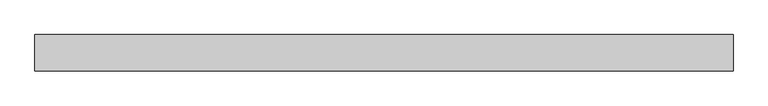
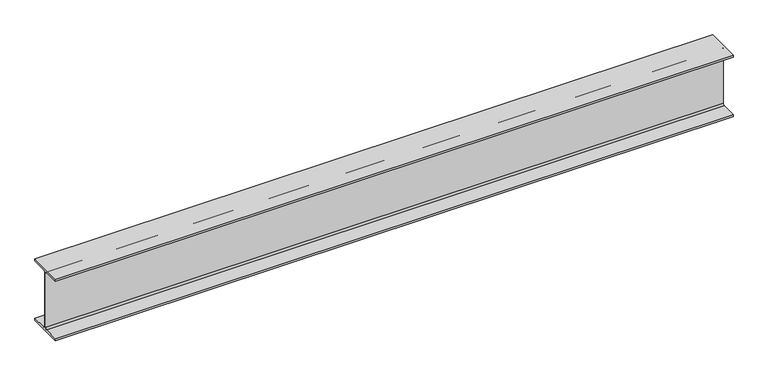
"""IFC4 building model written with IfcOpenShell, lengths in millimetres: beam geometry, Steel Beam_H-KSD3502 : H_SB_ASB_H-200x200x8x12."""

import ifcopenshell
import ifcopenshell.guid

model = None  # the IFC model being written
_history = None  # IfcOwnerHistory: only IFC2X3 demands one
_inside = {}  # id of a spatial element -> (the spatial element, [elements in it])
_under = {}  # id of a project, library or spatial element -> (it, [spatial elements below it])
_declared = {}  # id of a project -> (the project, [libraries it declares])
_typed = {}  # id of a type object -> (the type object, [elements of that type])
_made_of = {}  # id of a material, layer set ... -> (it, [elements and type objects made of it])


def new_model(schema):
    """Start an empty IFC model of exactly this schema.

    Asked for "IFC4X3", IfcOpenShell would pick the latest addendum, in which some entities
    have other attributes; the version numbers below select the first issue.
    IFC2X3 requires an IfcOwnerHistory on every rooted entity: one is made here for all.
    """
    global model, _history
    if schema == "IFC4X3":
        model = ifcopenshell.file(schema_version=(4, 3, 0, 0))
    else:
        model = ifcopenshell.file(schema=schema)
    _inside.clear()
    _under.clear()
    _declared.clear()
    _typed.clear()
    _made_of.clear()
    _history = None
    if model.schema == "IFC2X3":
        org = make("IfcOrganization", Name="unknown")
        user = make(
            "IfcPersonAndOrganization",
            ThePerson=make("IfcPerson", FamilyName="unknown"),
            TheOrganization=org,
        )
        app = make(
            "IfcApplication",
            ApplicationDeveloper=org,
            Version="unknown",
            ApplicationFullName="unknown",
            ApplicationIdentifier="unknown",
        )
        _history = make(
            "IfcOwnerHistory",
            OwningUser=user,
            OwningApplication=app,
            ChangeAction="ADDED",
            CreationDate=0,
        )
    return model


def make(cls, **values):
    """One entity of the class cls with the attributes given. An attribute that is None is left unset."""
    return model.create_entity(
        cls, **{name: value for name, value in values.items() if value is not None}
    )


def rooted(cls, **values):
    """An entity with a GlobalId (a new one), such as an element, a storey or a relation."""
    return make(cls, GlobalId=ifcopenshell.guid.new(), OwnerHistory=_history, **values)


def si_unit(unit_type, name, prefix=None):
    """IfcSIUnit, for example si_unit("LENGTHUNIT", "METRE", prefix="MILLI")."""
    return make("IfcSIUnit", UnitType=unit_type, Prefix=prefix, Name=name)


def assignment(units):
    """IfcUnitAssignment: the units of a project."""
    return None if units is None else make("IfcUnitAssignment", Units=units)


def point(xyz):
    """IfcCartesianPoint."""
    return None if xyz is None else make("IfcCartesianPoint", Coordinates=xyz)


def direction(xyz):
    """IfcDirection."""
    return None if xyz is None else make("IfcDirection", DirectionRatios=xyz)


def frame(location, z_axis=None, x_axis=None):
    """IfcAxis2Placement3D, a coordinate frame: its origin and axes. An axis left out is left unset."""
    return make(
        "IfcAxis2Placement3D",
        Location=point(location),
        Axis=direction(z_axis),
        RefDirection=direction(x_axis),
    )


def frame_2d(location, x_axis=None):
    """IfcAxis2Placement2D, a coordinate frame in the plane: its origin and x axis."""
    return make(
        "IfcAxis2Placement2D", Location=point(location), RefDirection=direction(x_axis)
    )


def origin():
    """The frame at (0, 0, 0) with its axes left unset."""
    return frame((0.0, 0.0, 0.0))


def place(relative_to, where):
    """IfcLocalPlacement: puts the frame where relative to a parent placement (None: the world)."""
    return make(
        "IfcLocalPlacement", PlacementRelTo=relative_to, RelativePlacement=where
    )


def context(
    kind, dimensions, precision=None, world=None, true_north=None, identifier=None
):
    """IfcGeometricRepresentationContext, for example the 3D "Model" context."""
    return make(
        "IfcGeometricRepresentationContext",
        ContextIdentifier=identifier,
        ContextType=kind,
        CoordinateSpaceDimension=dimensions,
        Precision=precision,
        WorldCoordinateSystem=world,
        TrueNorth=true_north,
    )


def project(units=None, contexts=None):
    """IfcProject with its units and contexts."""
    return rooted(
        "IfcProject",
        Name="project",
        RepresentationContexts=contexts,
        UnitsInContext=assignment(units),
    )


def spatial(cls, under=None, at=None, **own):
    """A site, building, storey or space (cls), placed at a placement, below another one or the project."""
    s = rooted(cls, ObjectPlacement=at, **own)
    if under is not None:
        _under.setdefault(under.id(), (under, []))[1].append(s)
    return s


def polyline(points):
    """IfcPolyline through the points."""
    return make("IfcPolyline", Points=[point(p) for p in points])


def circle_curve(where, radius):
    """IfcCircle in the frame where."""
    return make("IfcCircle", Position=where, Radius=radius)


def trimmed(basis, trim1, trim2, sense, master):
    """IfcTrimmedCurve: the piece of a basis curve between two trims."""
    return make(
        "IfcTrimmedCurve",
        BasisCurve=basis,
        Trim1=trim1,
        Trim2=trim2,
        SenseAgreement=sense,
        MasterRepresentation=master,
    )


def segment(curve, same_sense, transition):
    """IfcCompositeCurveSegment."""
    return make(
        "IfcCompositeCurveSegment",
        Transition=transition,
        SameSense=same_sense,
        ParentCurve=curve,
    )


def composite_curve(segments, self_intersect=None):
    """IfcCompositeCurve: segments joined end to end."""
    return make("IfcCompositeCurve", Segments=segments, SelfIntersect=self_intersect)


def outline(outer, holes=None, kind="AREA"):
    """IfcArbitraryClosedProfileDef: a profile drawn as a closed curve; with holes, ...WithVoids."""
    if holes is None:
        return make("IfcArbitraryClosedProfileDef", ProfileType=kind, OuterCurve=outer)
    return make(
        "IfcArbitraryProfileDefWithVoids",
        ProfileType=kind,
        OuterCurve=outer,
        InnerCurves=holes,
    )


def extrude(swept, where, along, depth):
    """IfcExtrudedAreaSolid: the profile swept, set in the frame where, extruded along a direction by depth."""
    return make(
        "IfcExtrudedAreaSolid",
        SweptArea=swept,
        Position=where,
        ExtrudedDirection=direction(along),
        Depth=depth,
    )


def shape(context_of_items, identifier, shape_type, items):
    """IfcShapeRepresentation: the items that make up one representation, for example the "Body"."""
    return make(
        "IfcShapeRepresentation",
        ContextOfItems=context_of_items,
        RepresentationIdentifier=identifier,
        RepresentationType=shape_type,
        Items=items,
    )


def source(mapping_origin, context_of_items, identifier, shape_type, items):
    """IfcRepresentationMap: a shape defined once, which mapped items show again and again."""
    return make(
        "IfcRepresentationMap",
        MappingOrigin=mapping_origin,
        MappedRepresentation=shape(context_of_items, identifier, shape_type, items),
    )


def transform(
    local_origin,
    x_axis=None,
    y_axis=None,
    z_axis=None,
    scale=None,
    scale2=None,
    scale3=None,
    uniform=True,
):
    """IfcCartesianTransformationOperator3D, or its non-uniform kind. x_axis, y_axis, z_axis: its Axis1, 2, 3."""
    if uniform:
        return make(
            "IfcCartesianTransformationOperator3D",
            Axis1=direction(x_axis),
            Axis2=direction(y_axis),
            LocalOrigin=point(local_origin),
            Scale=scale,
            Axis3=direction(z_axis),
        )
    return make(
        "IfcCartesianTransformationOperator3DnonUniform",
        Axis1=direction(x_axis),
        Axis2=direction(y_axis),
        LocalOrigin=point(local_origin),
        Scale=scale,
        Axis3=direction(z_axis),
        Scale2=scale2,
        Scale3=scale3,
    )


def mapped(mapping_source, mapping_target):
    """IfcMappedItem: shows the shape of a source again, moved by a transform."""
    return make(
        "IfcMappedItem", MappingSource=mapping_source, MappingTarget=mapping_target
    )


def made_of(thing, what):
    """Note that an element or type object is made of a material, layer set ...; save() writes the relation."""
    if what is not None:
        _made_of.setdefault(what.id(), (what, []))[1].append(thing)
    return thing


def element(
    cls,
    number,
    at=None,
    inside=None,
    cuts=None,
    type_object=None,
    material=None,
    context=None,
    identifier="Body",
    shape_type=None,
    held_by="IfcProductDefinitionShape",
    body=None,
    shapes=None,
    **own,
):
    """One element of the class cls, such as IfcWall. Its Tag is "e" and its number.

    at: its placement. inside: the storey or other place that contains it. cuts: it is an
    opening in that element (IfcRelVoidsElement). A single representation is given by context,
    identifier, shape_type and body (its items); several are given by shapes. held_by: the class
    of the entity that holds the representations. save() writes the other relations.
    """
    e = rooted(cls, Tag="e%d" % number, ObjectPlacement=at, **own)
    if body is not None:
        shapes = [shape(context, identifier, shape_type, body)]
    if shapes is not None:
        e.Representation = make(held_by, Representations=shapes)
    if inside is not None:
        _inside.setdefault(inside.id(), (inside, []))[1].append(e)
    if cuts is not None:
        rooted(
            "IfcRelVoidsElement", RelatingBuildingElement=cuts, RelatedOpeningElement=e
        )
    if type_object is not None:
        _typed.setdefault(type_object.id(), (type_object, []))[1].append(e)
    return made_of(e, material)


def aggregate(whole, parts):
    """IfcRelAggregates: a whole, such as a stair, and the parts it consists of."""
    return rooted("IfcRelAggregates", RelatingObject=whole, RelatedObjects=parts)


def save(model, path):
    """Write the relations noted so far, then the file.

    IfcRelAggregates (storeys below a building ...), IfcRelContainedInSpatialStructure (elements
    in a storey), IfcRelDefinesByType, IfcRelAssociatesMaterial and IfcRelDeclares: one each for
    every whole, place, type object, material and project.
    """
    for whole, parts in _under.values():
        aggregate(whole, parts)
    for where, things in _inside.values():
        rooted(
            "IfcRelContainedInSpatialStructure",
            RelatedElements=things,
            RelatingStructure=where,
        )
    for kind, things in _typed.values():
        rooted("IfcRelDefinesByType", RelatedObjects=things, RelatingType=kind)
    for what, things in _made_of.values():
        rooted("IfcRelAssociatesMaterial", RelatedObjects=things, RelatingMaterial=what)
    for by, libraries in _declared.values():
        rooted("IfcRelDeclares", RelatingContext=by, RelatedDefinitions=libraries)
    model.write(path)


def beam_1d8f39e2(model_context):
    return source(origin(), model_context, "Body", "SweptSolid", [
        extrude(outline(composite_curve([segment(polyline([(82.5, -141.5), (82.5, -151.7), (-82.5, -151.7), (-82.5, -141.5), (-11.9, -141.5)]), True, "CONTINUOUS"), segment(trimmed(circle_curve(frame_2d((-11.9, -132.6)), 8.9), [point((-11.9, -141.5))], [point((-3.0, -132.6))], True, "CARTESIAN"), True, "CONTINUOUS"), segment(polyline([(-3.0, -132.6), (-3.0, 132.6)]), True, "CONTINUOUS"), segment(trimmed(circle_curve(frame_2d((-11.9, 132.6)), 8.9), [point((-3.0, 132.6))], [point((-11.9, 141.5))], True, "CARTESIAN"), True, "CONTINUOUS"), segment(polyline([(-11.9, 141.5), (-82.5, 141.5), (-82.5, 151.7), (82.5, 151.7), (82.5, 141.5), (11.9, 141.5)]), True, "CONTINUOUS"), segment(trimmed(circle_curve(frame_2d((11.9, 132.6)), 8.9), [point((11.9, 141.5))], [point((3.0, 132.6))], True, "CARTESIAN"), True, "CONTINUOUS"), segment(polyline([(3.0, 132.6), (3.0, -132.6)]), True, "CONTINUOUS"), segment(trimmed(circle_curve(frame_2d((11.9, -132.6)), 8.9), [point((3.0, -132.6))], [point((11.9, -141.5))], True, "CARTESIAN"), True, "CONTINUOUS"), segment(polyline([(11.9, -141.5), (82.5, -141.5)]), True, "CONTINUOUS")], self_intersect=False)), frame((-1440.3194949, 0.0, 0.0), z_axis=(1.0, 0.0, 0.0), x_axis=(0.0, 1.0, 0.0)), (0.0, 0.0, 1.0), 3162.0635751),
    ])


if __name__ == "__main__":
    model = new_model("IFC4")
    model_context = context("Model", 3, world=origin())
    ifc_project = project(units=[si_unit("LENGTHUNIT", "METRE", prefix="MILLI")], contexts=[model_context])
    site = spatial("IfcSite", under=ifc_project)
    building = spatial("IfcBuilding", under=site)
    placement = place(None, origin())
    beam_shape = beam_1d8f39e2(model_context)
    element("IfcBeam", 1, ObjectType="Steel Beam_H-KSD3502 : H_SB_ASB_H-200x200x8x12", at=placement, inside=building, context=model_context, shape_type="MappedRepresentation", body=[
        mapped(beam_shape, transform((0.0, 0.0, 0.0), x_axis=(1.0, 0.0, 0.0), y_axis=(0.0, 1.0, 0.0), z_axis=(0.0, 0.0, 1.0))),
    ])
    save(model, "model.ifc")

# Revit data of these elements
# Type "Steel Beam_H-KSD3502 : H_SB_ASB_H-200x200x8x12"
#   Width = 20.0 cm
#   Web Thickness = 0.8 cm
#   Web Fillet = 1.3 cm
#   Warping Constant = 141376.0 cm⁶
#   Torsional Moment of Inertia = 26.2485 cm⁴
#   Torsional Modulus = 1.0 cm³
#   Section Area = 63.53 cm²
#   Plastic Modulus weak axis = 244.0 cm³
#   Plastic Modulus strong axis = 525.0 cm³
#   Perimeter = 1.16 m²/m
#   Nominal Weight = 49.90 kgf/m
#   Moment of Inertia weak axis = 1600.00 cm⁴
#   Moment of Inertia strong axis = 4720.00 cm⁴
#   Height = 20.0 cm
#   Flange Thickness = 1.2 cm
#   Elastic Modulus weak axis = 160.0 cm³
#   Elastic Modulus strong axis = 472.0 cm³
#   Centroid Vertical = 10.0 cm
#   Centroid Horizontal = 10.0 cm
#   Length [instance default] = 1.5240 m
#   Structural Material [instance default] = Steel, 45-345
#   Assembly Code = ""
# Element 1 (IfcBeam, "Steel Beam_H-KSD3502 : H_SB_ASB_H-200x200x8x12")
#   Structural Material = none
# Materials
#   "Steel, 45-345": class "Metal", colour RGB 189 187 185, transparency 0, Description = "Steel 345 MPa", Cost = 0
